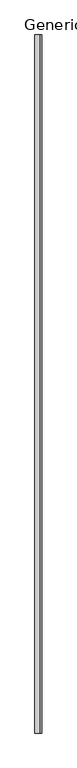
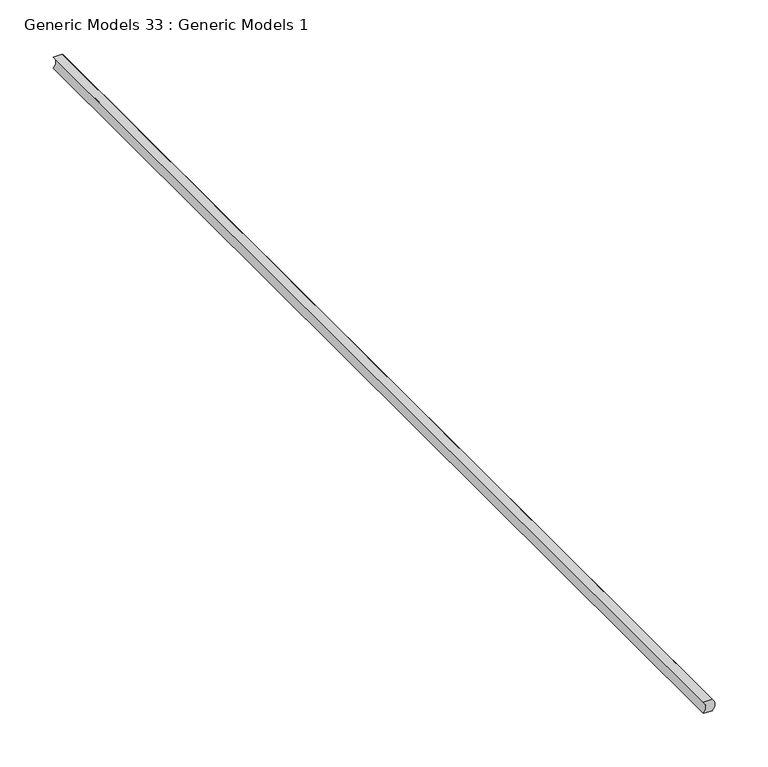
"""IFC4 building model written with IfcOpenShell, lengths in millimetres: proxy geometry, Generic Models 33 : Generic Models 1."""

import ifcopenshell
import ifcopenshell.guid

model = None  # the IFC model being written
_history = None  # IfcOwnerHistory: only IFC2X3 demands one
_inside = {}  # id of a spatial element -> (the spatial element, [elements in it])
_under = {}  # id of a project, library or spatial element -> (it, [spatial elements below it])
_declared = {}  # id of a project -> (the project, [libraries it declares])
_typed = {}  # id of a type object -> (the type object, [elements of that type])
_made_of = {}  # id of a material, layer set ... -> (it, [elements and type objects made of it])


def new_model(schema):
    """Start an empty IFC model of exactly this schema.

    Asked for "IFC4X3", IfcOpenShell would pick the latest addendum, in which some entities
    have other attributes; the version numbers below select the first issue.
    IFC2X3 requires an IfcOwnerHistory on every rooted entity: one is made here for all.
    """
    global model, _history
    if schema == "IFC4X3":
        model = ifcopenshell.file(schema_version=(4, 3, 0, 0))
    else:
        model = ifcopenshell.file(schema=schema)
    _inside.clear()
    _under.clear()
    _declared.clear()
    _typed.clear()
    _made_of.clear()
    _history = None
    if model.schema == "IFC2X3":
        org = make("IfcOrganization", Name="unknown")
        user = make(
            "IfcPersonAndOrganization",
            ThePerson=make("IfcPerson", FamilyName="unknown"),
            TheOrganization=org,
        )
        app = make(
            "IfcApplication",
            ApplicationDeveloper=org,
            Version="unknown",
            ApplicationFullName="unknown",
            ApplicationIdentifier="unknown",
        )
        _history = make(
            "IfcOwnerHistory",
            OwningUser=user,
            OwningApplication=app,
            ChangeAction="ADDED",
            CreationDate=0,
        )
    return model


def make(cls, **values):
    """One entity of the class cls with the attributes given. An attribute that is None is left unset."""
    return model.create_entity(
        cls, **{name: value for name, value in values.items() if value is not None}
    )


def rooted(cls, **values):
    """An entity with a GlobalId (a new one), such as an element, a storey or a relation."""
    return make(cls, GlobalId=ifcopenshell.guid.new(), OwnerHistory=_history, **values)


def si_unit(unit_type, name, prefix=None):
    """IfcSIUnit, for example si_unit("LENGTHUNIT", "METRE", prefix="MILLI")."""
    return make("IfcSIUnit", UnitType=unit_type, Prefix=prefix, Name=name)


def assignment(units):
    """IfcUnitAssignment: the units of a project."""
    return None if units is None else make("IfcUnitAssignment", Units=units)


def point(xyz):
    """IfcCartesianPoint."""
    return None if xyz is None else make("IfcCartesianPoint", Coordinates=xyz)


def direction(xyz):
    """IfcDirection."""
    return None if xyz is None else make("IfcDirection", DirectionRatios=xyz)


def frame(location, z_axis=None, x_axis=None):
    """IfcAxis2Placement3D, a coordinate frame: its origin and axes. An axis left out is left unset."""
    return make(
        "IfcAxis2Placement3D",
        Location=point(location),
        Axis=direction(z_axis),
        RefDirection=direction(x_axis),
    )


def frame_2d(location, x_axis=None):
    """IfcAxis2Placement2D, a coordinate frame in the plane: its origin and x axis."""
    return make(
        "IfcAxis2Placement2D", Location=point(location), RefDirection=direction(x_axis)
    )


def origin():
    """The frame at (0, 0, 0) with its axes left unset."""
    return frame((0.0, 0.0, 0.0))


def place(relative_to, where):
    """IfcLocalPlacement: puts the frame where relative to a parent placement (None: the world)."""
    return make(
        "IfcLocalPlacement", PlacementRelTo=relative_to, RelativePlacement=where
    )


def context(
    kind, dimensions, precision=None, world=None, true_north=None, identifier=None
):
    """IfcGeometricRepresentationContext, for example the 3D "Model" context."""
    return make(
        "IfcGeometricRepresentationContext",
        ContextIdentifier=identifier,
        ContextType=kind,
        CoordinateSpaceDimension=dimensions,
        Precision=precision,
        WorldCoordinateSystem=world,
        TrueNorth=true_north,
    )


def project(units=None, contexts=None):
    """IfcProject with its units and contexts."""
    return rooted(
        "IfcProject",
        Name="project",
        RepresentationContexts=contexts,
        UnitsInContext=assignment(units),
    )


def spatial(cls, under=None, at=None, **own):
    """A site, building, storey or space (cls), placed at a placement, below another one or the project."""
    s = rooted(cls, ObjectPlacement=at, **own)
    if under is not None:
        _under.setdefault(under.id(), (under, []))[1].append(s)
    return s


def polyline(points):
    """IfcPolyline through the points."""
    return make("IfcPolyline", Points=[point(p) for p in points])


def circle_curve(where, radius):
    """IfcCircle in the frame where."""
    return make("IfcCircle", Position=where, Radius=radius)


def trimmed(basis, trim1, trim2, sense, master):
    """IfcTrimmedCurve: the piece of a basis curve between two trims."""
    return make(
        "IfcTrimmedCurve",
        BasisCurve=basis,
        Trim1=trim1,
        Trim2=trim2,
        SenseAgreement=sense,
        MasterRepresentation=master,
    )


def segment(curve, same_sense, transition):
    """IfcCompositeCurveSegment."""
    return make(
        "IfcCompositeCurveSegment",
        Transition=transition,
        SameSense=same_sense,
        ParentCurve=curve,
    )


def composite_curve(segments, self_intersect=None):
    """IfcCompositeCurve: segments joined end to end."""
    return make("IfcCompositeCurve", Segments=segments, SelfIntersect=self_intersect)


def outline(outer, holes=None, kind="AREA"):
    """IfcArbitraryClosedProfileDef: a profile drawn as a closed curve; with holes, ...WithVoids."""
    if holes is None:
        return make("IfcArbitraryClosedProfileDef", ProfileType=kind, OuterCurve=outer)
    return make(
        "IfcArbitraryProfileDefWithVoids",
        ProfileType=kind,
        OuterCurve=outer,
        InnerCurves=holes,
    )


def extrude(swept, where, along, depth):
    """IfcExtrudedAreaSolid: the profile swept, set in the frame where, extruded along a direction by depth."""
    return make(
        "IfcExtrudedAreaSolid",
        SweptArea=swept,
        Position=where,
        ExtrudedDirection=direction(along),
        Depth=depth,
    )


def shape(context_of_items, identifier, shape_type, items):
    """IfcShapeRepresentation: the items that make up one representation, for example the "Body"."""
    return make(
        "IfcShapeRepresentation",
        ContextOfItems=context_of_items,
        RepresentationIdentifier=identifier,
        RepresentationType=shape_type,
        Items=items,
    )


def source(mapping_origin, context_of_items, identifier, shape_type, items):
    """IfcRepresentationMap: a shape defined once, which mapped items show again and again."""
    return make(
        "IfcRepresentationMap",
        MappingOrigin=mapping_origin,
        MappedRepresentation=shape(context_of_items, identifier, shape_type, items),
    )


def transform(
    local_origin,
    x_axis=None,
    y_axis=None,
    z_axis=None,
    scale=None,
    scale2=None,
    scale3=None,
    uniform=True,
):
    """IfcCartesianTransformationOperator3D, or its non-uniform kind. x_axis, y_axis, z_axis: its Axis1, 2, 3."""
    if uniform:
        return make(
            "IfcCartesianTransformationOperator3D",
            Axis1=direction(x_axis),
            Axis2=direction(y_axis),
            LocalOrigin=point(local_origin),
            Scale=scale,
            Axis3=direction(z_axis),
        )
    return make(
        "IfcCartesianTransformationOperator3DnonUniform",
        Axis1=direction(x_axis),
        Axis2=direction(y_axis),
        LocalOrigin=point(local_origin),
        Scale=scale,
        Axis3=direction(z_axis),
        Scale2=scale2,
        Scale3=scale3,
    )


def mapped(mapping_source, mapping_target):
    """IfcMappedItem: shows the shape of a source again, moved by a transform."""
    return make(
        "IfcMappedItem", MappingSource=mapping_source, MappingTarget=mapping_target
    )


def made_of(thing, what):
    """Note that an element or type object is made of a material, layer set ...; save() writes the relation."""
    if what is not None:
        _made_of.setdefault(what.id(), (what, []))[1].append(thing)
    return thing


def element(
    cls,
    number,
    at=None,
    inside=None,
    cuts=None,
    type_object=None,
    material=None,
    context=None,
    identifier="Body",
    shape_type=None,
    held_by="IfcProductDefinitionShape",
    body=None,
    shapes=None,
    **own,
):
    """One element of the class cls, such as IfcWall. Its Tag is "e" and its number.

    at: its placement. inside: the storey or other place that contains it. cuts: it is an
    opening in that element (IfcRelVoidsElement). A single representation is given by context,
    identifier, shape_type and body (its items); several are given by shapes. held_by: the class
    of the entity that holds the representations. save() writes the other relations.
    """
    e = rooted(cls, Tag="e%d" % number, ObjectPlacement=at, **own)
    if body is not None:
        shapes = [shape(context, identifier, shape_type, body)]
    if shapes is not None:
        e.Representation = make(held_by, Representations=shapes)
    if inside is not None:
        _inside.setdefault(inside.id(), (inside, []))[1].append(e)
    if cuts is not None:
        rooted(
            "IfcRelVoidsElement", RelatingBuildingElement=cuts, RelatedOpeningElement=e
        )
    if type_object is not None:
        _typed.setdefault(type_object.id(), (type_object, []))[1].append(e)
    return made_of(e, material)


def aggregate(whole, parts):
    """IfcRelAggregates: a whole, such as a stair, and the parts it consists of."""
    return rooted("IfcRelAggregates", RelatingObject=whole, RelatedObjects=parts)


def save(model, path):
    """Write the relations noted so far, then the file.

    IfcRelAggregates (storeys below a building ...), IfcRelContainedInSpatialStructure (elements
    in a storey), IfcRelDefinesByType, IfcRelAssociatesMaterial and IfcRelDeclares: one each for
    every whole, place, type object, material and project.
    """
    for whole, parts in _under.values():
        aggregate(whole, parts)
    for where, things in _inside.values():
        rooted(
            "IfcRelContainedInSpatialStructure",
            RelatedElements=things,
            RelatingStructure=where,
        )
    for kind, things in _typed.values():
        rooted("IfcRelDefinesByType", RelatedObjects=things, RelatingType=kind)
    for what, things in _made_of.values():
        rooted("IfcRelAssociatesMaterial", RelatedObjects=things, RelatingMaterial=what)
    for by, libraries in _declared.values():
        rooted("IfcRelDeclares", RelatingContext=by, RelatedDefinitions=libraries)
    model.write(path)


def generic_models_33_generic_models_1_2dc3aaa3(model_context):
    return source(origin(), model_context, "Body", "SweptSolid", [
        extrude(outline(composite_curve([segment(polyline([(2444.75, 49676.05), (2444.75, 49685.575)]), True, "CONTINUOUS"), segment(trimmed(circle_curve(frame_2d((2451.1, 49679.745519)), 8.620055), [point((2444.75, 49685.575))], [point((2457.45, 49685.575))], False, "CARTESIAN"), True, "CONTINUOUS"), segment(polyline([(2457.45, 49685.575), (2457.45, 49676.05)]), True, "CONTINUOUS"), segment(trimmed(circle_curve(frame_2d((2451.1, 49670.220519)), 8.620055), [point((2457.45, 49676.05))], [point((2444.75, 49676.05))], True, "CARTESIAN"), True, "CONTINUOUS")], self_intersect=False)), frame((0.0, 0.0, 0.0), z_axis=(0.0, 1.0, 0.0), x_axis=(0.0, 0.0, 1.0)), (0.0, 0.0, 1.0), 1219.2),
    ])


if __name__ == "__main__":
    model = new_model("IFC4")
    model_context = context("Model", 3, world=origin())
    ifc_project = project(units=[si_unit("LENGTHUNIT", "METRE", prefix="MILLI")], contexts=[model_context])
    site = spatial("IfcSite", under=ifc_project)
    building = spatial("IfcBuilding", under=site)
    placement = place(None, origin())
    generic_models_33_generic_models_1_shape = generic_models_33_generic_models_1_2dc3aaa3(model_context)
    element("IfcBuildingElementProxy", 1, Name="Generic Models 33 : Generic Models 1", ObjectType="Generic Models 33 : Generic Models 1", at=placement, inside=building, context=model_context, shape_type="MappedRepresentation", body=[
        mapped(generic_models_33_generic_models_1_shape, transform((0.0, 0.0, 0.0), x_axis=(1.0, 0.0, 0.0), y_axis=(0.0, 1.0, 0.0), z_axis=(0.0, 0.0, 1.0))),
    ])
    save(model, "model.ifc")

# Revit data of these elements
# Element 1 (IfcBuildingElementProxy, "Generic Models 33 : Generic Models 1")
#   Materials on its faces: "ACOUSTICAL SEALANT"
# Materials
#   "ACOUSTICAL SEALANT": class "Unassigned", colour RGB 120 120 120, transparency 0, Cost = 0
